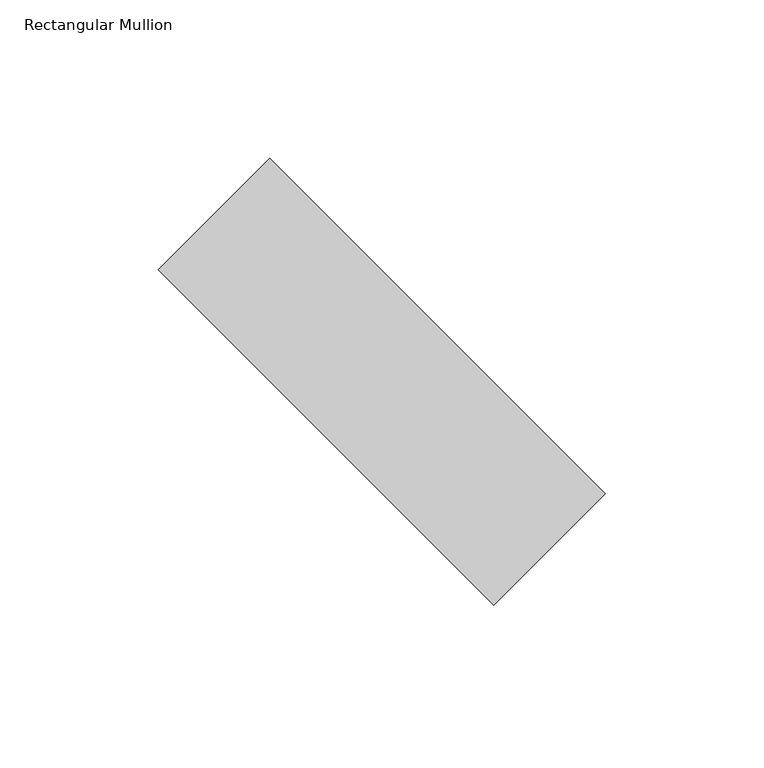
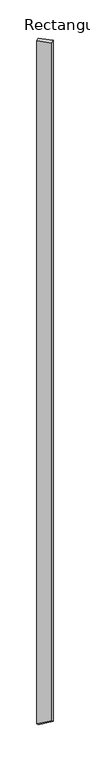
"""IFC4 building model written with IfcOpenShell, lengths in millimetres: member geometry, Rectangular Mullion : tilted mullions."""

from ifc_helpers import new_model, si_unit, origin, place, context, project, spatial, faceted_brep, source, transform, mapped, element, save


def rectangular_mullion_61da3b18(model_context):
    return source(origin(), model_context, "Body", "Brep", [
        faceted_brep([(-35.3553391, 70.7106781, 0.0), (-70.7106781, 35.3553391, 0.0), (35.3553391, -70.7106781, 0.0), (70.7106781, -35.3553391, 0.0), (-35.3553391, 70.7106781, -8054.2583644), (-70.7106781, 35.3553391, -8009.214773), (35.3553391, -70.7106781, -7944.101995), (70.7106781, -35.3553391, -7989.1455864)], [[[0, 1, 2, 3]], [[1, 0, 4, 5]], [[2, 1, 5, 6]], [[3, 2, 6, 7]], [[0, 3, 7, 4]], [[4, 7, 6, 5]]]),
    ])


if __name__ == "__main__":
    model = new_model("IFC4")
    model_context = context("Model", 3, world=origin())
    ifc_project = project(units=[si_unit("LENGTHUNIT", "METRE", prefix="MILLI")], contexts=[model_context])
    site = spatial("IfcSite", under=ifc_project)
    building = spatial("IfcBuilding", under=site)
    placement = place(None, origin())
    rectangular_mullion_shape = rectangular_mullion_61da3b18(model_context)
    element("IfcMember", 1, ObjectType="Rectangular Mullion : tilted mullions", at=placement, inside=building, context=model_context, shape_type="MappedRepresentation", body=[
        mapped(rectangular_mullion_shape, transform((0.0, 0.0, 0.0), x_axis=(1.0, 0.0, 0.0), y_axis=(0.0, 1.0, 0.0), z_axis=(0.0, 0.0, 1.0))),
    ])
    save(model, "model.ifc")

# Revit data of these elements
# Type "Rectangular Mullion : tilted mullions"
#   built-in parameter 1007304 = 0.492126 (stored number, unit not read)
#   built-in parameter 1007301 = 0.082021 (stored number, unit not read)
#   built-in parameter 1007300 = 0.082021 (stored number, unit not read)
# Element 1 (IfcMember, "Rectangular Mullion : tilted mullions")
#   Materials on its faces: "Aluminum"
# Materials
#   "Aluminum": class "Metal", colour RGB 244 244 244, transparency 0, Description = "Aluminum 6061", Cost = 0
